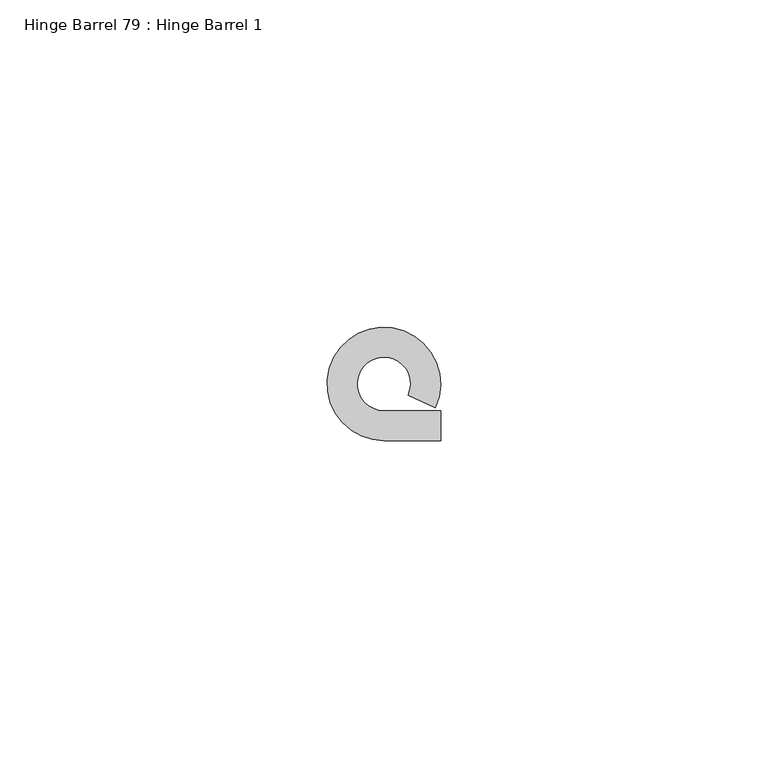
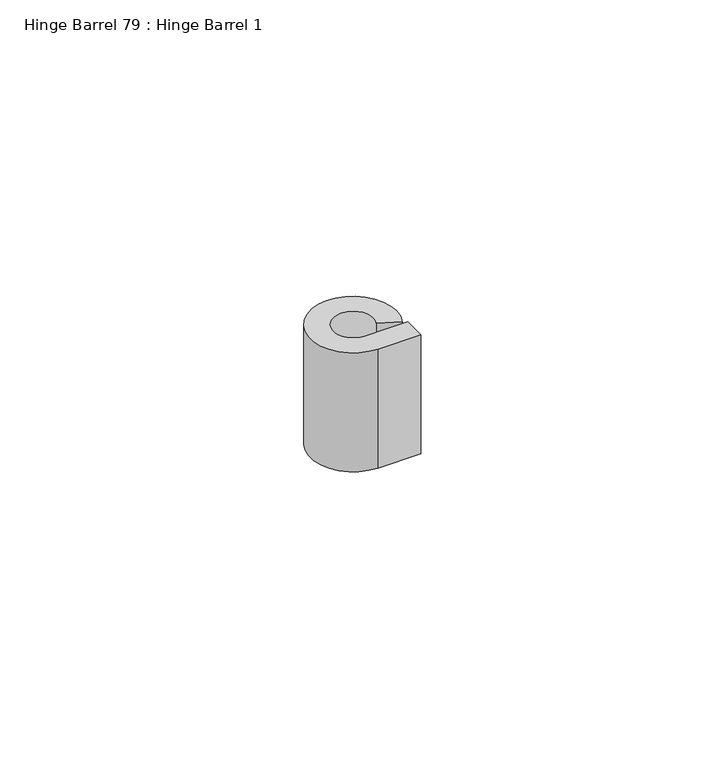
"""IFC4 building model written with IfcOpenShell, lengths in millimetres: proxy geometry, Hinge Barrel 79 : Hinge Barrel 1."""

from ifc_helpers import new_model, si_unit, point, frame, frame_2d, origin, place, context, project, spatial, polyline, circle_curve, trimmed, segment, composite_curve, outline, extrude, source, transform, mapped, element, save


def hinge_barrel_79_hinge_barrel_1_4fbccd9d(model_context):
    return source(origin(), model_context, "Body", "SweptSolid", [
        extrude(outline(composite_curve([segment(polyline([(587323.2214739, -531780.6943841), (587327.7934739, -531780.6943841), (587327.7934739, -531785.2584466), (587319.1320739, -531785.2584466)]), True, "CONTINUOUS"), segment(trimmed(circle_curve(frame_2d((587319.1320739, -531776.6049841)), 8.6534625), [point((587319.1320739, -531785.2584466))], [point((587326.986084, -531780.2377433))], False, "CARTESIAN"), True, "CONTINUOUS"), segment(polyline([(587326.986084, -531780.2377433), (587322.8436736, -531778.321731)]), True, "CONTINUOUS"), segment(trimmed(circle_curve(frame_2d((587319.1320739, -531776.6049841)), 4.0894), [point((587322.8436736, -531778.321731))], [point((587319.1320739, -531780.6943841))], True, "CARTESIAN"), True, "CONTINUOUS"), segment(polyline([(587319.1320739, -531780.6943841), (587323.2214739, -531780.6943841)]), True, "CONTINUOUS")], self_intersect=False)), frame((0.0, 0.0, 1936.75), z_axis=(0.0, 0.0, 1.0), x_axis=(1.0, 0.0, 0.0)), (0.0, 0.0, 1.0), 25.4),
    ])


if __name__ == "__main__":
    model = new_model("IFC4")
    model_context = context("Model", 3, world=origin())
    ifc_project = project(units=[si_unit("LENGTHUNIT", "METRE", prefix="MILLI")], contexts=[model_context])
    site = spatial("IfcSite", under=ifc_project)
    building = spatial("IfcBuilding", under=site)
    placement = place(None, origin())
    hinge_barrel_79_hinge_barrel_1_shape = hinge_barrel_79_hinge_barrel_1_4fbccd9d(model_context)
    element("IfcBuildingElementProxy", 1, Name="Hinge Barrel 79 : Hinge Barrel 1", ObjectType="Hinge Barrel 79 : Hinge Barrel 1", at=placement, inside=building, context=model_context, shape_type="MappedRepresentation", body=[
        mapped(hinge_barrel_79_hinge_barrel_1_shape, transform((0.0, 0.0, 0.0), x_axis=(1.0, 0.0, 0.0), y_axis=(0.0, 1.0, 0.0), z_axis=(0.0, 0.0, 1.0))),
    ])
    save(model, "model.ifc")

# Revit data of these elements
# Element 1 (IfcBuildingElementProxy, "Hinge Barrel 79 : Hinge Barrel 1")
#   Materials on its faces: "6\"X6\" WELD-ON STL BUTT HINGE"
# Materials
#   "6\"X6\" WELD-ON STL BUTT HINGE": class "Metal", colour RGB 189 187 185, transparency 0, Description = "Carbon steel", Cost = 0
